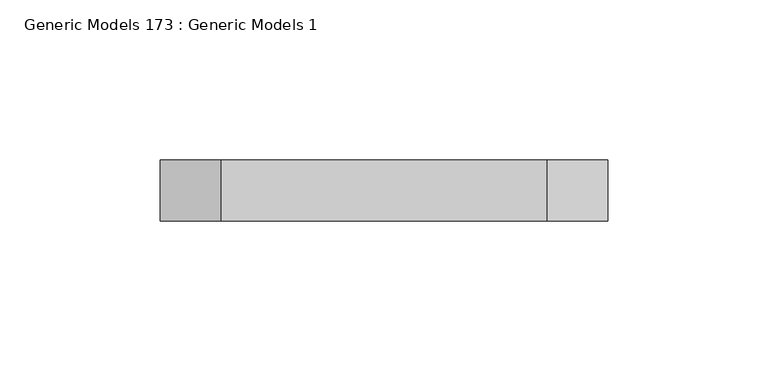
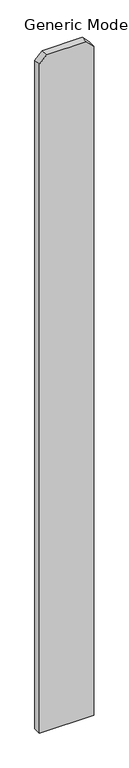
"""IFC4 building model written with IfcOpenShell, lengths in millimetres: proxy geometry, Generic Models 173 : Generic Models 1."""

from ifc_helpers import new_model, si_unit, frame, origin, place, context, project, spatial, polyline, outline, extrude, source, transform, mapped, element, save


def generic_models_173_generic_models_1_d081218f(model_context):
    return source(origin(), model_context, "Body", "SweptSolid", [
        extrude(outline(polyline([(76.2, -248438.9875), (1885.95, -248438.9875), (1905.0, -248458.0375), (1905.0, -248559.6375), (1885.95, -248578.6875), (76.2, -248578.6875), (76.2, -248438.9875)])), frame((0.0, 547.6875, 0.0), z_axis=(0.0, 1.0, 0.0), x_axis=(0.0, 0.0, 1.0)), (0.0, 0.0, 1.0), 19.05),
    ])


if __name__ == "__main__":
    model = new_model("IFC4")
    model_context = context("Model", 3, world=origin())
    ifc_project = project(units=[si_unit("LENGTHUNIT", "METRE", prefix="MILLI")], contexts=[model_context])
    site = spatial("IfcSite", under=ifc_project)
    building = spatial("IfcBuilding", under=site)
    placement = place(None, origin())
    generic_models_173_generic_models_1_shape = generic_models_173_generic_models_1_d081218f(model_context)
    element("IfcBuildingElementProxy", 1, Name="Generic Models 173 : Generic Models 1", ObjectType="Generic Models 173 : Generic Models 1", at=placement, inside=building, context=model_context, shape_type="MappedRepresentation", body=[
        mapped(generic_models_173_generic_models_1_shape, transform((0.0, 0.0, 0.0), x_axis=(1.0, 0.0, 0.0), y_axis=(0.0, 1.0, 0.0), z_axis=(0.0, 0.0, 1.0))),
    ])
    save(model, "model.ifc")

# Revit data of these elements
# Element 1 (IfcBuildingElementProxy, "Generic Models 173 : Generic Models 1")
#   Materials on its faces: "VERTICAL 1X6 CEDAR PLANKS W/ CLEAR WOOD SEALER"
# Materials
#   "VERTICAL 1X6 CEDAR PLANKS W/ CLEAR WOOD SEALER": class "Wood", colour RGB 234 198 147, transparency 0, Description = "Pinus Echinata", Cost = 0
